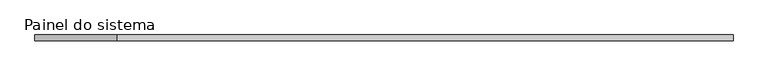
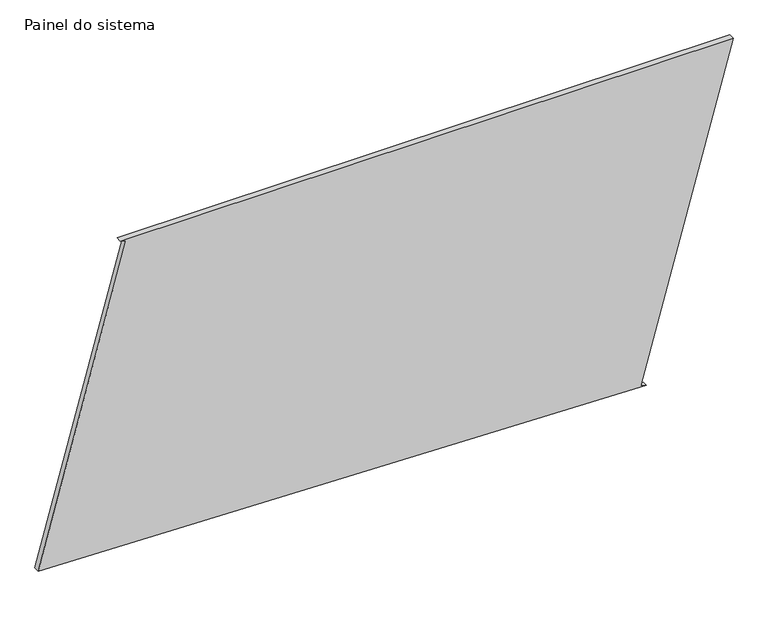
"""IFC4 building model written with IfcOpenShell, lengths in millimetres: plate geometry, Painel do sistema : Envidraçado."""

from ifc_helpers import new_model, si_unit, frame, origin, place, context, project, spatial, polyline, outline, extrude, source, transform, mapped, element, save


def painel_do_sistema_e874d16d(model_context):
    return source(origin(), model_context, "Body", "SweptSolid", [
        extrude(outline(polyline([(0.0, 1124.5702484), (6.6310485, 1100.4657012), (1452.3431664, 1498.1743645), (1452.3431664, -1144.0957), (1445.7121178, -1119.9911528), (70.9770358, -1498.1743645), (0.0, 1124.5702484)])), frame((0.0, 24.5, 0.0), z_axis=(0.0, 1.0, 0.0), x_axis=(0.0, 0.0, 1.0)), (0.0, 0.0, 1.0), 25.0),
    ])


if __name__ == "__main__":
    model = new_model("IFC4")
    model_context = context("Model", 3, world=origin())
    ifc_project = project(units=[si_unit("LENGTHUNIT", "METRE", prefix="MILLI")], contexts=[model_context])
    site = spatial("IfcSite", under=ifc_project)
    building = spatial("IfcBuilding", under=site)
    placement = place(None, origin())
    painel_do_sistema_shape = painel_do_sistema_e874d16d(model_context)
    element("IfcPlate", 1, ObjectType="Painel do sistema : Envidraçado", at=placement, inside=building, context=model_context, shape_type="MappedRepresentation", body=[
        mapped(painel_do_sistema_shape, transform((0.0, 0.0, 0.0), x_axis=(1.0, 0.0, 0.0), y_axis=(0.0, 1.0, 0.0), z_axis=(0.0, 0.0, 1.0))),
    ])
    save(model, "model.ifc")

# Revit data of these elements
# Type "Painel do sistema : Envidraçado"
#   Construction Type Id = "GSP4R"
#   Analytic Construction = "Vidraça única Pilkington 1/8 pol"
#   Visual Light Transmittance = 0.9
#   Solar Heat Gain Coefficient = 0.86
#   Heat Transfer Coefficient (U) = 6.7069 W/(m²·K)
# Element 1 (IfcPlate, "Painel do sistema : Envidraçado")
#   Materials on its faces: "Vidro"
# Materials
#   "Vidro": class "Vidro", colour RGB 0 128 192, transparency 0.9, Description = "Vidro de sílica", Cost = 0
